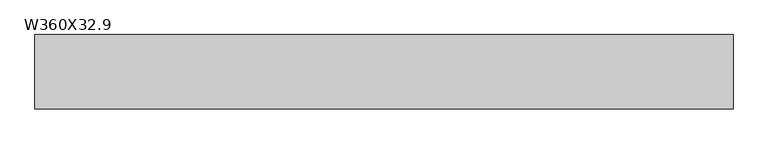
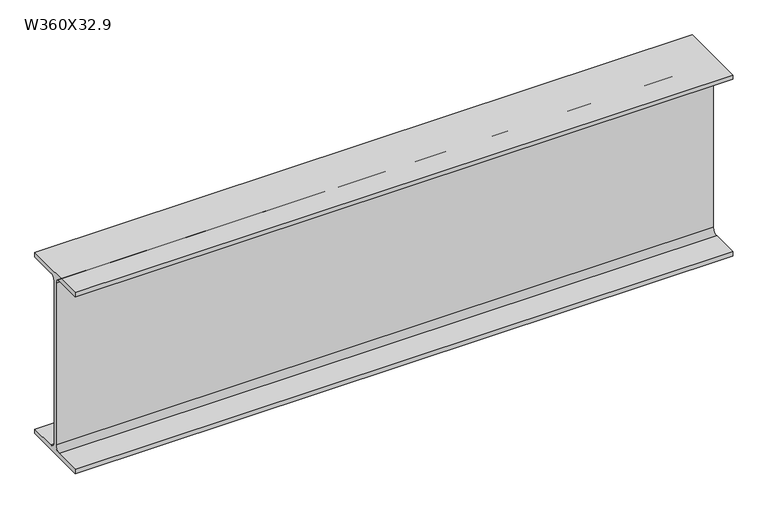
"""IFC4 building model written with IfcOpenShell, lengths in millimetres: beam geometry, M_W Shapes : W360X32.9."""

from ifc_helpers import new_model, si_unit, point, frame, frame_2d, origin, place, context, project, spatial, polyline, circle_curve, trimmed, segment, composite_curve, outline, extrude, source, transform, mapped, element, save


def w360x32_9_112d7f2e(model_context):
    return source(origin(), model_context, "Body", "SweptSolid", [
        extrude(outline(composite_curve([segment(polyline([(63.5, -165.49), (63.5, -174.0), (-63.5, -174.0), (-63.5, -165.49), (-13.11, -165.49)]), True, "CONTINUOUS"), segment(trimmed(circle_curve(frame_2d((-13.11, -155.3)), 10.19), [point((-13.11, -165.49))], [point((-2.92, -155.3))], True, "CARTESIAN"), True, "CONTINUOUS"), segment(polyline([(-2.92, -155.3), (-2.92, 155.3)]), True, "CONTINUOUS"), segment(trimmed(circle_curve(frame_2d((-13.11, 155.3)), 10.19), [point((-2.92, 155.3))], [point((-13.11, 165.49))], True, "CARTESIAN"), True, "CONTINUOUS"), segment(polyline([(-13.11, 165.49), (-63.5, 165.49), (-63.5, 174.0), (63.5, 174.0), (63.5, 165.49), (13.11, 165.49)]), True, "CONTINUOUS"), segment(trimmed(circle_curve(frame_2d((13.11, 155.3)), 10.19), [point((13.11, 165.49))], [point((2.92, 155.3))], True, "CARTESIAN"), True, "CONTINUOUS"), segment(polyline([(2.92, 155.3), (2.92, -155.3)]), True, "CONTINUOUS"), segment(trimmed(circle_curve(frame_2d((13.11, -155.3)), 10.19), [point((2.92, -155.3))], [point((13.11, -165.49))], True, "CARTESIAN"), True, "CONTINUOUS"), segment(polyline([(13.11, -165.49), (63.5, -165.49)]), True, "CONTINUOUS")], self_intersect=False)), frame((-597.3, 0.0, 0.0), z_axis=(1.0, 0.0, 0.0), x_axis=(0.0, 1.0, 0.0)), (0.0, 0.0, 1.0), 1194.6),
    ])


if __name__ == "__main__":
    model = new_model("IFC4")
    model_context = context("Model", 3, world=origin())
    ifc_project = project(units=[si_unit("LENGTHUNIT", "METRE", prefix="MILLI")], contexts=[model_context])
    site = spatial("IfcSite", under=ifc_project)
    building = spatial("IfcBuilding", under=site)
    placement = place(None, origin())
    w360x32_9_shape = w360x32_9_112d7f2e(model_context)
    element("IfcBeam", 1, ObjectType="M_W Shapes : W360X32.9", at=placement, inside=building, context=model_context, shape_type="MappedRepresentation", body=[
        mapped(w360x32_9_shape, transform((0.0, 0.0, 0.0), x_axis=(1.0, 0.0, 0.0), y_axis=(0.0, 1.0, 0.0), z_axis=(0.0, 0.0, 1.0))),
    ])
    save(model, "model.ifc")

# Revit data of these elements
# Project information
#   Название организации = "Organization Name"
#   Описание организации = "Organization Description"
#   Наименование здания = "Building Name"
#   Дата утверждения проекта = "Issue Date"
#   Статус проекта = "Project Status"
#   Заказчик = "Client Name"
#   Адрес проекта = "Enter address here\nAddress Line 2"
#   Наименование проекта = "Project Name"
#   Номер проекта = "Project Number"
# Type "M_W Shapes : W360X32.9"
#   Section Name Key = "W360X32.9"
#   Width = 12.7 cm
#   Web Thickness = 0.584 cm
#   Web Fillet = 1.019 cm
#   Warping Constant = 84300.0 cm⁶
#   Torsional Moment of Inertia = 8.66 cm⁴
#   Section Area = 41.9 cm²
#   Plastic Modulus weak axis = 71.9 cm³
#   Plastic Modulus strong axis = 544.0 cm³
#   Perimeter = 1.18 m²/m
#   Nominal Weight = 32.90 kgf/m
#   Moment of Inertia weak axis = 291.00 cm⁴
#   Moment of Inertia strong axis = 8280.00 cm⁴
#   Height = 34.8 cm
#   Flange Thickness = 0.851 cm
#   Elastic Modulus weak axis = 45.9 cm³
#   Elastic Modulus strong axis = 475.0 cm³
#   Clear Web Height = 29.5 cm
#   Centroid Vertical = 17.4 cm
#   Centroid Horizontal = 6.35 cm
#   Bolt Spacing = 6.99 cm
#   Length [instance default] = 1500 mm
#   Structural Material [instance default] = Steel ASTM A992
# Element 1 (IfcBeam, "M_W Shapes : W360X32.9")
#   Length = 1194.6 mm
#   Materials on its faces: "Steel ASTM A992"
# Materials
#   "Steel ASTM A992": class "Metal", colour RGB 203 203 203, transparency 0, Description = "Structural steel 50ksi", Cost = 0
